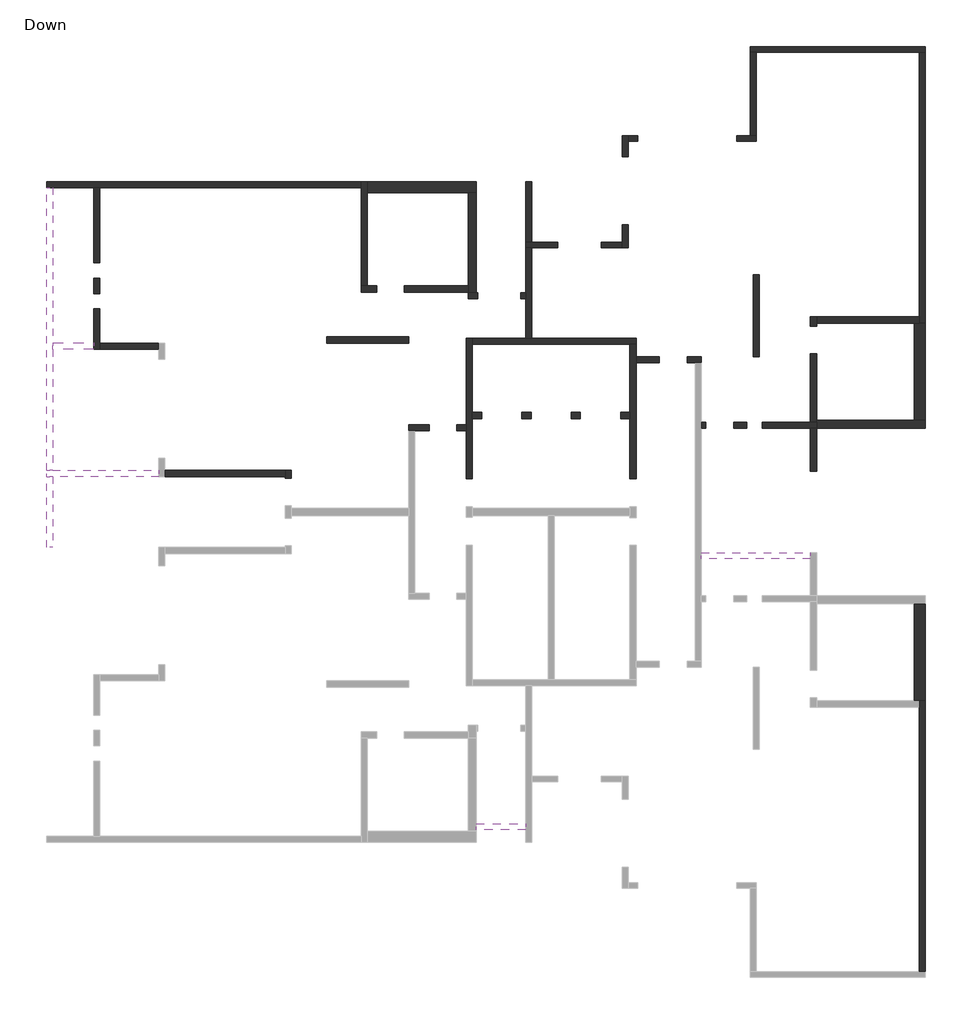
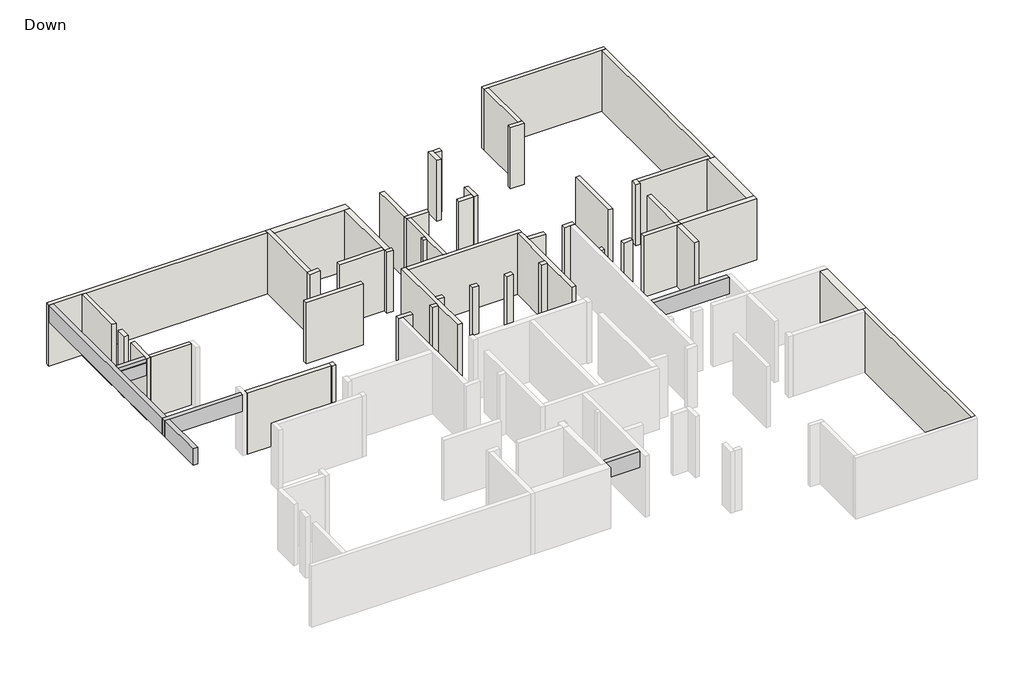
# One storey, part 2 of 2: 49 walls, 6 beams.
"""IFC4 building model written with IfcOpenShell, lengths in millimetres."""

import ifcopenshell
import ifcopenshell.guid

model = None  # the IFC model being written
_history = None  # IfcOwnerHistory: only IFC2X3 demands one
_inside = {}  # id of a spatial element -> (the spatial element, [elements in it])
_under = {}  # id of a project, library or spatial element -> (it, [spatial elements below it])
_declared = {}  # id of a project -> (the project, [libraries it declares])
_typed = {}  # id of a type object -> (the type object, [elements of that type])
_made_of = {}  # id of a material, layer set ... -> (it, [elements and type objects made of it])


def new_model(schema):
    """Start an empty IFC model of exactly this schema.

    Asked for "IFC4X3", IfcOpenShell would pick the latest addendum, in which some entities
    have other attributes; the version numbers below select the first issue.
    IFC2X3 requires an IfcOwnerHistory on every rooted entity: one is made here for all.
    """
    global model, _history
    if schema == "IFC4X3":
        model = ifcopenshell.file(schema_version=(4, 3, 0, 0))
    else:
        model = ifcopenshell.file(schema=schema)
    _inside.clear()
    _under.clear()
    _declared.clear()
    _typed.clear()
    _made_of.clear()
    _history = None
    if model.schema == "IFC2X3":
        org = make("IfcOrganization", Name="unknown")
        user = make(
            "IfcPersonAndOrganization",
            ThePerson=make("IfcPerson", FamilyName="unknown"),
            TheOrganization=org,
        )
        app = make(
            "IfcApplication",
            ApplicationDeveloper=org,
            Version="unknown",
            ApplicationFullName="unknown",
            ApplicationIdentifier="unknown",
        )
        _history = make(
            "IfcOwnerHistory",
            OwningUser=user,
            OwningApplication=app,
            ChangeAction="ADDED",
            CreationDate=0,
        )
    return model


def make(cls, **values):
    """One entity of the class cls with the attributes given. An attribute that is None is left unset."""
    return model.create_entity(
        cls, **{name: value for name, value in values.items() if value is not None}
    )


def rooted(cls, **values):
    """An entity with a GlobalId (a new one), such as an element, a storey or a relation."""
    return make(cls, GlobalId=ifcopenshell.guid.new(), OwnerHistory=_history, **values)


def si_unit(unit_type, name, prefix=None):
    """IfcSIUnit, for example si_unit("LENGTHUNIT", "METRE", prefix="MILLI")."""
    return make("IfcSIUnit", UnitType=unit_type, Prefix=prefix, Name=name)


def assignment(units):
    """IfcUnitAssignment: the units of a project."""
    return None if units is None else make("IfcUnitAssignment", Units=units)


def point(xyz):
    """IfcCartesianPoint."""
    return None if xyz is None else make("IfcCartesianPoint", Coordinates=xyz)


def direction(xyz):
    """IfcDirection."""
    return None if xyz is None else make("IfcDirection", DirectionRatios=xyz)


def frame(location, z_axis=None, x_axis=None):
    """IfcAxis2Placement3D, a coordinate frame: its origin and axes. An axis left out is left unset."""
    return make(
        "IfcAxis2Placement3D",
        Location=point(location),
        Axis=direction(z_axis),
        RefDirection=direction(x_axis),
    )


def origin():
    """The frame at (0, 0, 0) with its axes left unset."""
    return frame((0.0, 0.0, 0.0))


def place(relative_to, where):
    """IfcLocalPlacement: puts the frame where relative to a parent placement (None: the world)."""
    return make(
        "IfcLocalPlacement", PlacementRelTo=relative_to, RelativePlacement=where
    )


def context(
    kind, dimensions, precision=None, world=None, true_north=None, identifier=None
):
    """IfcGeometricRepresentationContext, for example the 3D "Model" context."""
    return make(
        "IfcGeometricRepresentationContext",
        ContextIdentifier=identifier,
        ContextType=kind,
        CoordinateSpaceDimension=dimensions,
        Precision=precision,
        WorldCoordinateSystem=world,
        TrueNorth=true_north,
    )


def project(units=None, contexts=None):
    """IfcProject with its units and contexts."""
    return rooted(
        "IfcProject",
        Name="project",
        RepresentationContexts=contexts,
        UnitsInContext=assignment(units),
    )


def spatial(cls, under=None, at=None, **own):
    """A site, building, storey or space (cls), placed at a placement, below another one or the project."""
    s = rooted(cls, ObjectPlacement=at, **own)
    if under is not None:
        _under.setdefault(under.id(), (under, []))[1].append(s)
    return s


def polyline(points):
    """IfcPolyline through the points."""
    return make("IfcPolyline", Points=[point(p) for p in points])


def outline(outer, holes=None, kind="AREA"):
    """IfcArbitraryClosedProfileDef: a profile drawn as a closed curve; with holes, ...WithVoids."""
    if holes is None:
        return make("IfcArbitraryClosedProfileDef", ProfileType=kind, OuterCurve=outer)
    return make(
        "IfcArbitraryProfileDefWithVoids",
        ProfileType=kind,
        OuterCurve=outer,
        InnerCurves=holes,
    )


def extrude(swept, where, along, depth):
    """IfcExtrudedAreaSolid: the profile swept, set in the frame where, extruded along a direction by depth."""
    return make(
        "IfcExtrudedAreaSolid",
        SweptArea=swept,
        Position=where,
        ExtrudedDirection=direction(along),
        Depth=depth,
    )


def faces_of(points, faces, orient=None, outer=None):
    """IfcFace entities. A face is a list of loops; a loop is a list of indices into points, from 0.

    orient and outer hold one flag for each loop. By default every Orientation is true, the
    first loop of a face is its IfcFaceOuterBound and the others are IfcFaceBound.
    """
    made = []
    for i, loops in enumerate(faces):
        bounds = []
        for j, loop in enumerate(loops):
            is_outer = j == 0 if outer is None else outer[i][j]
            bounds.append(
                make(
                    "IfcFaceOuterBound" if is_outer else "IfcFaceBound",
                    Bound=make("IfcPolyLoop", Polygon=[points[k] for k in loop]),
                    Orientation=True if orient is None else orient[i][j],
                )
            )
        made.append(make("IfcFace", Bounds=bounds))
    return made


def faceted_brep(points, faces, orient=None, outer=None, voids=None):
    """IfcFacetedBrep: a solid bounded by flat faces; with voids (closed shells), ...WithVoids."""
    shared = [point(p) for p in points]
    hull = make("IfcClosedShell", CfsFaces=faces_of(shared, faces, orient, outer))
    if voids is None:
        return make("IfcFacetedBrep", Outer=hull)
    return make(
        "IfcFacetedBrepWithVoids",
        Outer=hull,
        Voids=[
            make(cls, CfsFaces=faces_of(shared, fs, o, b)) for cls, fs, o, b in voids
        ],
    )


def shape(context_of_items, identifier, shape_type, items):
    """IfcShapeRepresentation: the items that make up one representation, for example the "Body"."""
    return make(
        "IfcShapeRepresentation",
        ContextOfItems=context_of_items,
        RepresentationIdentifier=identifier,
        RepresentationType=shape_type,
        Items=items,
    )


def made_of(thing, what):
    """Note that an element or type object is made of a material, layer set ...; save() writes the relation."""
    if what is not None:
        _made_of.setdefault(what.id(), (what, []))[1].append(thing)
    return thing


def element(
    cls,
    number,
    at=None,
    inside=None,
    cuts=None,
    type_object=None,
    material=None,
    context=None,
    identifier="Body",
    shape_type=None,
    held_by="IfcProductDefinitionShape",
    body=None,
    shapes=None,
    **own,
):
    """One element of the class cls, such as IfcWall. Its Tag is "e" and its number.

    at: its placement. inside: the storey or other place that contains it. cuts: it is an
    opening in that element (IfcRelVoidsElement). A single representation is given by context,
    identifier, shape_type and body (its items); several are given by shapes. held_by: the class
    of the entity that holds the representations. save() writes the other relations.
    """
    e = rooted(cls, Tag="e%d" % number, ObjectPlacement=at, **own)
    if body is not None:
        shapes = [shape(context, identifier, shape_type, body)]
    if shapes is not None:
        e.Representation = make(held_by, Representations=shapes)
    if inside is not None:
        _inside.setdefault(inside.id(), (inside, []))[1].append(e)
    if cuts is not None:
        rooted(
            "IfcRelVoidsElement", RelatingBuildingElement=cuts, RelatedOpeningElement=e
        )
    if type_object is not None:
        _typed.setdefault(type_object.id(), (type_object, []))[1].append(e)
    return made_of(e, material)


def aggregate(whole, parts):
    """IfcRelAggregates: a whole, such as a stair, and the parts it consists of."""
    return rooted("IfcRelAggregates", RelatingObject=whole, RelatedObjects=parts)


def save(model, path):
    """Write the relations noted so far, then the file.

    IfcRelAggregates (storeys below a building ...), IfcRelContainedInSpatialStructure (elements
    in a storey), IfcRelDefinesByType, IfcRelAssociatesMaterial and IfcRelDeclares: one each for
    every whole, place, type object, material and project.
    """
    for whole, parts in _under.values():
        aggregate(whole, parts)
    for where, things in _inside.values():
        rooted(
            "IfcRelContainedInSpatialStructure",
            RelatedElements=things,
            RelatingStructure=where,
        )
    for kind, things in _typed.values():
        rooted("IfcRelDefinesByType", RelatedObjects=things, RelatingType=kind)
    for what, things in _made_of.values():
        rooted("IfcRelAssociatesMaterial", RelatedObjects=things, RelatingMaterial=what)
    for by, libraries in _declared.values():
        rooted("IfcRelDeclares", RelatingContext=by, RelatedDefinitions=libraries)
    model.write(path)


model = new_model("IFC4")

# Units and contexts
model_context = context("Model", 3, world=origin())
ifc_project = project(units=[si_unit("LENGTHUNIT", "METRE", prefix="MILLI")], contexts=[model_context])

# Site, building, storey
site = spatial("IfcSite", under=ifc_project)
building = spatial("IfcBuilding", under=site)
storey = spatial("IfcBuildingStorey", under=building, Name="Down", Elevation=0.0)

# Beams
placement = place(None, origin())
element("IfcBeam", 1, ObjectType="Concrete Rectengular Beam : 20/80", at=placement, inside=storey, context=model_context, shape_type="Brep", body=[
    faceted_brep([(7776.7577342, 15926.4707233, 3000.0), (7776.7577342, 16126.4707233, 3000.0), (4344.3623691, 16126.4707233, 3000.0), (4144.3623691, 16126.4707233, 3000.0), (4144.3623691, 15926.4707233, 3000.0), (4344.3623691, 15926.4707233, 3000.0), (7776.7577342, 16126.4707233, 2810.0), (7776.7577342, 16126.4707233, 2200.0), (4344.3623691, 16126.4707233, 2200.0), (4144.3623691, 16126.4707233, 2200.0), (7776.7577342, 15926.4707233, 2200.0), (4344.3623691, 15926.4707233, 2200.0), (4144.3623691, 15926.4707233, 2200.0)], [[[0, 1, 2, 3, 4, 5]], [[1, 6, 7, 8, 9, 3, 2]], [[7, 10, 11, 12, 9, 8]], [[10, 0, 5, 4, 12, 11]], [[1, 0, 10, 7, 6]], [[4, 3, 9, 12]]]),
])
element("IfcBeam", 2, ObjectType="Concrete Rectengular Beam : 20/80", at=placement, inside=storey, context=model_context, shape_type="Brep", body=[
    faceted_brep([(4344.3623691, 25280.6199284, 3000.0), (4144.3623691, 25280.6199284, 3000.0), (4144.3623691, 16126.4707233, 3000.0), (4344.3623691, 16126.4707233, 3000.0), (4344.3623691, 20073.0459905, 3000.0), (4344.3623691, 20253.0459905, 3000.0), (4344.3623691, 25280.6199284, 2200.0), (4344.3623691, 25280.6199284, 2810.0), (4344.3623691, 16126.4707233, 2810.0), (4344.3623691, 16126.4707233, 2200.0), (4344.3623691, 20058.0459905, 2200.0), (4344.3623691, 20258.0459905, 2200.0), (4144.3623691, 25280.6199284, 2200.0), (4144.3623691, 16126.4707233, 2200.0)], [[[0, 1, 2, 3, 4, 5]], [[6, 7, 0, 5, 4, 3, 8, 9, 10, 11]], [[12, 6, 11, 10, 9, 13]], [[1, 12, 13, 2]], [[1, 0, 7, 6, 12]], [[3, 2, 13, 9, 8]]]),
])
element("IfcBeam", 3, ObjectType="Concrete Rectengular Beam : 20/80", at=placement, inside=storey, context=model_context, shape_type="SweptSolid", body=[
    extrude(outline(polyline([(20258.0459905, 2200.0), (20058.0459905, 2200.0), (20058.0459905, 2810.0), (20073.0459905, 2810.0), (20073.0459905, 3000.0), (20253.0459905, 3000.0), (20253.0459905, 2810.0), (20258.0459905, 2810.0), (20258.0459905, 2200.0)])), frame((4344.3623691, 0.0, 0.0), z_axis=(1.0, 0.0, 0.0), x_axis=(0.0, 1.0, 0.0)), (0.0, 0.0, 1.0), 1331.6661672),
])
element("IfcBeam", 4, ObjectType="Concrete Rectengular Beam : 20/80", at=placement, inside=storey, context=model_context, shape_type="SweptSolid", body=[
    extrude(outline(polyline([(4144.3623691, 15926.4707233), (4344.3623691, 15926.4707233), (4344.3623691, 13635.0363012), (4144.3623691, 13635.0363012), (4144.3623691, 15926.4707233)])), frame((0.0, 0.0, 2200.0), z_axis=(0.0, 0.0, 1.0), x_axis=(1.0, 0.0, 0.0)), (0.0, 0.0, 1.0), 800.0),
])
element("IfcBeam", 5, ObjectType="Concrete Rectengular Beam : 20/80", at=placement, inside=storey, context=model_context, shape_type="Brep", body=[
    faceted_brep([(25344.8278571, 13464.5588264, 3000.0), (25344.8278571, 13264.5588264, 3000.0), (28875.6979001, 13264.5588264, 3000.0), (28875.6979001, 13464.5588264, 3000.0), (25344.8278571, 13464.5588264, 2200.0), (28875.6979001, 13464.5588264, 2200.0), (25344.8278571, 13264.5588264, 2200.0), (28875.6979001, 13264.5588264, 2200.0), (25344.8278571, 13264.5588264, 2810.0), (28875.6979001, 13264.5588264, 2810.0)], [[[0, 1, 2, 3]], [[4, 0, 3, 5]], [[6, 4, 5, 7]], [[1, 8, 6, 7, 9, 2]], [[1, 0, 4, 6, 8]], [[3, 2, 9, 7, 5]]]),
])
element("IfcBeam", 6, ObjectType="Concrete Rectengular Beam : 20/80", at=placement, inside=storey, context=model_context, shape_type="Brep", body=[
    faceted_brep([(19662.6522503, 4492.2283899, 3000.0), (19662.6522503, 4692.2283899, 3000.0), (18051.1049523, 4692.2283899, 3000.0), (18051.1049523, 4492.2283899, 3000.0), (19662.6522503, 4492.2283899, 2200.0), (18051.1049523, 4492.2283899, 2200.0), (19662.6522503, 4692.2283899, 2200.0), (18051.1049523, 4692.2283899, 2200.0), (19662.6522503, 4692.2283899, 2810.0), (18051.1049523, 4692.2283899, 2810.0)], [[[0, 1, 2, 3]], [[4, 0, 3, 5]], [[6, 4, 5, 7]], [[1, 8, 6, 7, 9, 2]], [[1, 0, 4, 6, 8]], [[3, 2, 9, 7, 5]]]),
])

# Walls
element("IfcWall", 7, ObjectType="19", at=placement, inside=storey, context=model_context, shape_type="Brep", body=[
    faceted_brep([(32597.3840453, 29852.2723415, 0.0), (26934.7329615, 29852.2723415, 0.0), (26934.7329615, 29852.2723415, 2810.0), (26934.7329615, 29852.2723415, 3000.0), (32597.3840453, 29852.2723415, 3000.0), (32597.3840453, 29662.2723415, 0.0), (32597.3840453, 29662.2723415, 3000.0), (32407.3840453, 29662.2723415, 3000.0), (27124.7329615, 29662.2723415, 3000.0), (26934.7329615, 29662.2723415, 3000.0), (26934.7329615, 29662.2723415, 0.0), (27124.7329615, 29662.2723415, 0.0), (32407.3840453, 29662.2723415, 0.0)], [[[0, 1, 2, 3, 4]], [[5, 6, 7, 8, 9, 10, 11, 12]], [[1, 0, 5, 12, 11, 10]], [[4, 3, 9, 8, 7, 6]], [[3, 2, 1, 10, 9]], [[0, 4, 6, 5]]]),
])
element("IfcWall", 8, ObjectType="19", at=placement, inside=storey, context=model_context, shape_type="Brep", body=[
    faceted_brep([(14329.4188071, 25470.6199284, 0.0), (4143.9417549, 25470.6199284, 0.0), (4143.9417549, 25470.6199284, 3000.0), (14329.4188071, 25470.6199284, 3000.0), (14329.4188071, 25280.6199284, 0.0), (14329.4188071, 25280.6199284, 2810.0), (14329.4188071, 25280.6199284, 3000.0), (5866.0285364, 25280.6199284, 3000.0), (5676.0285364, 25280.6199284, 3000.0), (4344.3623691, 25280.6199284, 3000.0), (4143.9417549, 25280.6199284, 3000.0), (4143.9417549, 25280.6199284, 0.0), (5676.0285364, 25280.6199284, 0.0), (5866.0285364, 25280.6199284, 0.0)], [[[0, 1, 2, 3]], [[4, 5, 6, 7, 8, 9, 10, 11, 12, 13]], [[1, 0, 4, 13, 12, 11]], [[2, 1, 11, 10]], [[3, 2, 10, 9, 8, 7, 6]], [[0, 3, 6, 5, 4]]]),
])
element("IfcWall", 9, ObjectType="19", at=placement, inside=storey, context=model_context, shape_type="Brep", body=[
    faceted_brep([(5676.0285364, 25280.6199284, 0.0), (5676.0285364, 22851.8697843, 0.0), (5676.0285364, 22851.8697843, 2810.0), (5676.0285364, 22851.8697843, 3000.0), (5676.0285364, 25280.6199284, 3000.0), (5676.0285364, 25280.6199284, 2810.0), (5866.0285364, 25280.6199284, 0.0), (5866.0285364, 25280.6199284, 2810.0), (5866.0285364, 25280.6199284, 3000.0), (5866.0285364, 22851.8697843, 3000.0), (5866.0285364, 22851.8697843, 2810.0), (5866.0285364, 22851.8697843, 0.0), (5681.0285364, 22851.8697843, 3000.0)], [[[0, 1, 2, 3, 4, 5]], [[6, 7, 8, 9, 10, 11]], [[1, 0, 6, 11]], [[3, 2, 1, 11, 10, 9, 12]], [[4, 3, 12, 9, 8]], [[0, 5, 4, 8, 7, 6]]]),
])
element("IfcWall", 10, ObjectType="19", at=placement, inside=storey, context=model_context, shape_type="Brep", body=[
    faceted_brep([(5676.0285364, 22352.6390151, 0.0), (5676.0285364, 21853.4082459, 0.0), (5676.0285364, 21853.4082459, 2810.0), (5676.0285364, 21853.4082459, 3000.0), (5676.0285364, 22352.6390151, 3000.0), (5676.0285364, 22352.6390151, 2810.0), (5866.0285364, 22352.6390151, 0.0), (5866.0285364, 22352.6390151, 2810.0), (5866.0285364, 22352.6390151, 3000.0), (5866.0285364, 21853.4082459, 3000.0), (5866.0285364, 21853.4082459, 2810.0), (5866.0285364, 21853.4082459, 0.0), (5681.0285364, 21853.4082459, 3000.0), (5681.0285364, 22352.6390151, 3000.0)], [[[0, 1, 2, 3, 4, 5]], [[6, 7, 8, 9, 10, 11]], [[1, 0, 6, 11]], [[3, 2, 1, 11, 10, 9, 12]], [[4, 3, 12, 9, 8, 13]], [[0, 5, 4, 13, 8, 7, 6]]]),
])
element("IfcWall", 11, ObjectType="19", at=placement, inside=storey, context=model_context, shape_type="Brep", body=[
    faceted_brep([(5676.0285364, 21354.1774766, 0.0), (5676.0285364, 20058.0459905, 0.0), (5676.0285364, 20058.0459905, 2810.0), (5676.0285364, 20058.0459905, 3000.0), (5676.0285364, 20073.0459905, 3000.0), (5676.0285364, 20253.0459905, 3000.0), (5676.0285364, 21354.1774766, 3000.0), (5676.0285364, 21354.1774766, 2810.0), (5866.0285364, 21354.1774766, 0.0), (5866.0285364, 21354.1774766, 2810.0), (5866.0285364, 21354.1774766, 3000.0), (5866.0285364, 20248.0459905, 3000.0), (5866.0285364, 20058.0459905, 3000.0), (5866.0285364, 20058.0459905, 0.0), (5866.0285364, 20248.0459905, 0.0), (5681.0285364, 21354.1774766, 3000.0)], [[[0, 1, 2, 3, 4, 5, 6, 7]], [[8, 9, 10, 11, 12, 13, 14]], [[1, 0, 8, 14, 13]], [[6, 5, 4, 3, 12, 11, 10, 15]], [[0, 7, 6, 15, 10, 9, 8]], [[3, 2, 1, 13, 12]]]),
])
element("IfcWall", 12, ObjectType="19", at=placement, inside=storey, context=model_context, shape_type="Brep", body=[
    faceted_brep([(26934.7329615, 29662.2723415, 0.0), (26934.7329615, 26971.6500261, 0.0), (26934.7329615, 26971.6500261, 2810.0), (26934.7329615, 26971.6500261, 3000.0), (26934.7329615, 29662.2723415, 3000.0), (27124.7329615, 29662.2723415, 0.0), (27124.7329615, 29662.2723415, 2810.0), (27124.7329615, 29662.2723415, 3000.0), (27124.7329615, 26971.6500261, 3000.0), (27124.7329615, 26971.6500261, 0.0)], [[[0, 1, 2, 3, 4]], [[5, 6, 7, 8, 9]], [[1, 0, 5, 9]], [[4, 3, 8, 7]], [[0, 4, 7, 6, 5]], [[3, 2, 1, 9, 8]]]),
])
element("IfcWall", 13, ObjectType="19", at=placement, inside=storey, context=model_context, shape_type="Brep", body=[
    faceted_brep([(27124.7329615, 26971.6500261, 0.0), (26934.7329615, 26971.6500261, 0.0), (26490.0221434, 26971.6500261, 0.0), (26490.0221434, 26971.6500261, 2810.0), (26490.0221434, 26971.6500261, 3000.0), (26934.7329615, 26971.6500261, 3000.0), (27124.7329615, 26971.6500261, 3000.0), (27124.7329615, 26781.6500261, 0.0), (27124.7329615, 26781.6500261, 2810.0), (27124.7329615, 26781.6500261, 3000.0), (26490.0221434, 26781.6500261, 3000.0), (26490.0221434, 26781.6500261, 2810.0), (26490.0221434, 26781.6500261, 0.0)], [[[0, 1, 2, 3, 4, 5, 6]], [[7, 8, 9, 10, 11, 12]], [[2, 1, 0, 7, 12]], [[4, 3, 2, 12, 11, 10]], [[6, 5, 4, 10, 9]], [[0, 6, 9, 8, 7]]]),
])
element("IfcWall", 14, ObjectType="19", at=placement, inside=storey, context=model_context, shape_type="Brep", body=[
    faceted_brep([(23288.1042531, 26971.6500261, 0.0), (22974.0986592, 26971.6500261, 0.0), (22974.0986592, 26971.6500261, 3000.0), (23288.1042531, 26971.6500261, 3000.0), (23288.1042531, 26971.6500261, 2810.0), (23288.1042531, 26781.6500261, 0.0), (23288.1042531, 26781.6500261, 2810.0), (23288.1042531, 26781.6500261, 3000.0), (22974.0986592, 26781.6500261, 3000.0), (22974.0986592, 26781.6500261, 2810.0), (22974.0986592, 26781.6500261, 0.0)], [[[0, 1, 2, 3, 4]], [[5, 6, 7, 8, 9, 10]], [[1, 0, 5, 10]], [[3, 2, 8, 7]], [[0, 4, 3, 7, 6, 5]], [[2, 1, 10, 9, 8]]]),
])
element("IfcWall", 15, ObjectType="19", at=placement, inside=storey, context=model_context, shape_type="Brep", body=[
    faceted_brep([(22784.0986592, 26971.6500261, 0.0), (22784.0986592, 26281.8797734, 0.0), (22784.0986592, 26281.8797734, 2810.0), (22784.0986592, 26281.8797734, 3000.0), (22784.0986592, 26971.6500261, 3000.0), (22784.0986592, 26971.6500261, 2810.0), (22974.0986592, 26971.6500261, 0.0), (22974.0986592, 26971.6500261, 3000.0), (22974.0986592, 26781.6500261, 3000.0), (22974.0986592, 26281.8797734, 3000.0), (22974.0986592, 26281.8797734, 2810.0), (22974.0986592, 26281.8797734, 0.0), (22974.0986592, 26781.6500261, 0.0)], [[[0, 1, 2, 3, 4, 5]], [[6, 7, 8, 9, 10, 11, 12]], [[1, 0, 6, 12, 11]], [[3, 2, 1, 11, 10, 9]], [[4, 3, 9, 8, 7]], [[0, 5, 4, 7, 6]]]),
])
element("IfcWall", 16, ObjectType="19", at=placement, inside=storey, context=model_context, shape_type="Brep", body=[
    faceted_brep([(22784.6890098, 24081.620059, 0.0), (22784.6890098, 23519.8470094, 0.0), (22784.6890098, 23329.8470094, 0.0), (22784.6890098, 23329.8470094, 3000.0), (22784.6890098, 23519.8470094, 3000.0), (22784.6890098, 24081.620059, 3000.0), (22784.6890098, 24081.620059, 2810.0), (22974.6890098, 24081.620059, 0.0), (22974.6890098, 24081.620059, 2810.0), (22974.6890098, 24081.620059, 3000.0), (22974.6890098, 23329.8470094, 3000.0), (22974.6890098, 23329.8470094, 2810.0), (22974.6890098, 23329.8470094, 0.0)], [[[0, 1, 2, 3, 4, 5, 6]], [[7, 8, 9, 10, 11, 12]], [[2, 1, 0, 7, 12]], [[5, 4, 3, 10, 9]], [[0, 6, 5, 9, 8, 7]], [[3, 2, 12, 11, 10]]]),
])
element("IfcWall", 17, ObjectType="19", at=placement, inside=storey, context=model_context, shape_type="Brep", body=[
    faceted_brep([(22784.6890098, 23519.8470094, 0.0), (22104.3264087, 23519.8470094, 0.0), (22104.3264087, 23519.8470094, 2810.0), (22104.3264087, 23519.8470094, 3000.0), (22784.6890098, 23519.8470094, 3000.0), (22784.6890098, 23519.8470094, 2810.0), (22784.6890098, 23329.8470094, 0.0), (22784.6890098, 23329.8470094, 3000.0), (22104.3264087, 23329.8470094, 3000.0), (22104.3264087, 23329.8470094, 2810.0), (22104.3264087, 23329.8470094, 0.0)], [[[0, 1, 2, 3, 4, 5]], [[6, 7, 8, 9, 10]], [[1, 0, 6, 10]], [[3, 2, 1, 10, 9, 8]], [[4, 3, 8, 7]], [[0, 5, 4, 7, 6]]]),
])
element("IfcWall", 18, ObjectType="19", at=placement, inside=storey, context=model_context, shape_type="Brep", body=[
    faceted_brep([(20702.4284964, 23519.8470094, 0.0), (19852.6522503, 23519.8470094, 0.0), (19662.6522503, 23519.8470094, 0.0), (19662.6522503, 23519.8470094, 3000.0), (19852.6522503, 23519.8470094, 3000.0), (20702.4284964, 23519.8470094, 3000.0), (20702.4284964, 23519.8470094, 2810.0), (20702.4284964, 23329.8470094, 0.0), (20702.4284964, 23329.8470094, 2810.0), (20702.4284964, 23329.8470094, 3000.0), (19852.6522503, 23329.8470094, 3000.0), (19662.6522503, 23329.8470094, 3000.0), (19662.6522503, 23329.8470094, 0.0), (19852.6522503, 23329.8470094, 0.0)], [[[0, 1, 2, 3, 4, 5, 6]], [[7, 8, 9, 10, 11, 12, 13]], [[2, 1, 0, 7, 13, 12]], [[5, 4, 3, 11, 10, 9]], [[0, 6, 5, 9, 8, 7]], [[3, 2, 12, 11]]]),
])
element("IfcWall", 19, ObjectType="19", at=placement, inside=storey, context=model_context, shape_type="Brep", body=[
    faceted_brep([(19852.6522503, 23519.8470094, 0.0), (19852.6522503, 25470.811948, 0.0), (19852.6522503, 25470.811948, 2810.0), (19852.6522503, 25470.811948, 3000.0), (19852.6522503, 23519.8470094, 3000.0), (19852.6522503, 23519.8470094, 2810.0), (19662.6522503, 23519.8470094, 0.0), (19662.6522503, 23519.8470094, 3000.0), (19662.6522503, 24869.2786346, 3000.0), (19662.6522503, 25470.811948, 3000.0), (19662.6522503, 25470.811948, 2810.0), (19662.6522503, 25470.811948, 0.0)], [[[0, 1, 2, 3, 4, 5]], [[6, 7, 8, 9, 10, 11]], [[1, 0, 6, 11]], [[3, 2, 1, 11, 10, 9]], [[4, 3, 9, 8, 7]], [[0, 5, 4, 7, 6]]]),
])
element("IfcWall", 20, ObjectType="19", at=placement, inside=storey, context=model_context, shape_type="Brep", body=[
    faceted_brep([(32407.3840453, 29662.2723415, 0.0), (32407.3840453, 21099.9399072, 0.0), (32407.3840453, 20899.9399072, 0.0), (32407.3840453, 20899.9399072, 3000.0), (32407.3840453, 21099.9399072, 3000.0), (32407.3840453, 29662.2723415, 3000.0), (32407.3840453, 29662.2723415, 2810.0), (32597.3840453, 29662.2723415, 0.0), (32597.3840453, 29662.2723415, 3000.0), (32597.3840453, 20899.9399072, 3000.0), (32597.3840453, 20899.9399072, 0.0)], [[[0, 1, 2, 3, 4, 5, 6]], [[7, 8, 9, 10]], [[2, 1, 0, 7, 10]], [[5, 4, 3, 9, 8]], [[0, 6, 5, 8, 7]], [[3, 2, 10, 9]]]),
])
element("IfcWall", 21, ObjectType="19", at=placement, inside=storey, context=model_context, shape_type="Brep", body=[
    faceted_brep([(5866.0285364, 20058.0459905, 0.0), (7776.7577342, 20058.0459905, 0.0), (7776.7577342, 20058.0459905, 2810.0), (7776.7577342, 20058.0459905, 3000.0), (5866.0285364, 20058.0459905, 3000.0), (5866.0285364, 20248.0459905, 0.0), (5866.0285364, 20248.0459905, 2810.0), (5866.0285364, 20248.0459905, 3000.0), (7776.7577342, 20248.0459905, 3000.0), (7776.7577342, 20248.0459905, 0.0)], [[[0, 1, 2, 3, 4]], [[5, 6, 7, 8, 9]], [[1, 0, 5, 9]], [[4, 3, 8, 7]], [[0, 4, 7, 6, 5]], [[3, 2, 1, 9, 8]]]),
])
element("IfcWall", 22, ObjectType="19", at=placement, inside=storey, context=model_context, shape_type="Brep", body=[
    faceted_brep([(11878.6856136, 16126.4707233, 0.0), (11878.6856136, 15926.4707233, 0.0), (11878.6856136, 15877.7643004, 0.0), (11878.6856136, 15877.7643004, 2810.0), (11878.6856136, 15877.7643004, 3000.0), (11878.6856136, 15926.4707233, 3000.0), (11878.6856136, 16126.4707233, 3000.0), (12068.6856136, 16126.4707233, 0.0), (12068.6856136, 16126.4707233, 2810.0), (12068.6856136, 16126.4707233, 3000.0), (12068.6856136, 15877.7643004, 3000.0), (12068.6856136, 15877.7643004, 2810.0), (12068.6856136, 15877.7643004, 0.0)], [[[0, 1, 2, 3, 4, 5, 6]], [[7, 8, 9, 10, 11, 12]], [[2, 1, 0, 7, 12]], [[4, 3, 2, 12, 11, 10]], [[6, 5, 4, 10, 9]], [[0, 6, 9, 8, 7]]]),
])
element("IfcWall", 23, ObjectType="19", at=placement, inside=storey, context=model_context, shape_type="Brep", body=[
    faceted_brep([(17801.1049523, 21688.6523235, 0.0), (18101.9290458, 21688.6523235, 0.0), (18101.9290458, 21688.6523235, 2810.0), (18101.9290458, 21688.6523235, 3000.0), (17801.1049523, 21688.6523235, 3000.0), (17801.1049523, 21688.6523235, 2810.0), (17801.1049523, 21878.6523235, 0.0), (17801.1049523, 21878.6523235, 3000.0), (18051.1049523, 21878.6523235, 3000.0), (18101.9290458, 21878.6523235, 3000.0), (18101.9290458, 21878.6523235, 2810.0), (18101.9290458, 21878.6523235, 0.0), (18051.1049523, 21878.6523235, 0.0)], [[[0, 1, 2, 3, 4, 5]], [[6, 7, 8, 9, 10, 11, 12]], [[1, 0, 6, 12, 11]], [[3, 2, 1, 11, 10, 9]], [[4, 3, 9, 8, 7]], [[0, 5, 4, 7, 6]]]),
])
element("IfcWall", 24, ObjectType="19", at=placement, inside=storey, context=model_context, shape_type="Brep", body=[
    faceted_brep([(19501.7092875, 21688.6523235, 0.0), (19662.6522503, 21688.6523235, 0.0), (19662.6522503, 21688.6523235, 2810.0), (19662.6522503, 21688.6523235, 3000.0), (19501.7092875, 21688.6523235, 3000.0), (19501.7092875, 21688.6523235, 2810.0), (19501.7092875, 21878.6523235, 0.0), (19501.7092875, 21878.6523235, 2810.0), (19501.7092875, 21878.6523235, 3000.0), (19662.6522503, 21878.6523235, 3000.0), (19662.6522503, 21878.6523235, 2810.0), (19662.6522503, 21878.6523235, 0.0)], [[[0, 1, 2, 3, 4, 5]], [[6, 7, 8, 9, 10, 11]], [[1, 0, 6, 11]], [[4, 3, 9, 8]], [[0, 5, 4, 8, 7, 6]], [[3, 2, 1, 11, 10, 9]]]),
])
element("IfcWall", 25, ObjectType="19", at=placement, inside=storey, context=model_context, shape_type="Brep", body=[
    faceted_brep([(19662.6522503, 23329.8470094, 0.0), (19662.6522503, 21878.6523235, 0.0), (19662.6522503, 21688.6523235, 0.0), (19662.6522503, 20409.5793039, 0.0), (19662.6522503, 20409.5793039, 2810.0), (19662.6522503, 20409.5793039, 3000.0), (19662.6522503, 21688.6523235, 3000.0), (19662.6522503, 21878.6523235, 3000.0), (19662.6522503, 23329.8470094, 3000.0), (19852.6522503, 23329.8470094, 0.0), (19852.6522503, 23329.8470094, 2810.0), (19852.6522503, 23329.8470094, 3000.0), (19852.6522503, 20409.5793039, 3000.0), (19852.6522503, 20409.5793039, 2810.0), (19852.6522503, 20409.5793039, 0.0)], [[[0, 1, 2, 3, 4, 5, 6, 7, 8]], [[9, 10, 11, 12, 13, 14]], [[3, 2, 1, 0, 9, 14]], [[8, 7, 6, 5, 12, 11]], [[0, 8, 11, 10, 9]], [[5, 4, 3, 14, 13, 12]]]),
])
element("IfcWall", 26, ObjectType="19", at=placement, inside=storey, context=model_context, shape_type="Brep", body=[
    faceted_brep([(32597.3840453, -100.765317, 0.0), (32597.3840453, 8661.5671173, 0.0), (32597.3840453, 8661.5671173, 3000.0), (32597.3840453, -100.765317, 3000.0), (32407.3840453, -100.765317, 0.0), (32407.3840453, -100.765317, 2810.0), (32407.3840453, -100.765317, 3000.0), (32407.3840453, 8461.5671173, 3000.0), (32407.3840453, 8661.5671173, 3000.0), (32407.3840453, 8661.5671173, 0.0), (32407.3840453, 8461.5671173, 0.0)], [[[0, 1, 2, 3]], [[4, 5, 6, 7, 8, 9, 10]], [[1, 0, 4, 10, 9]], [[3, 2, 8, 7, 6]], [[0, 3, 6, 5, 4]], [[2, 1, 9, 8]]]),
])
element("IfcWall", 27, ObjectType="20", at=placement, inside=storey, context=model_context, shape_type="Brep", body=[
    faceted_brep([(14529.4188071, 22100.4193798, 0.0), (14529.4188071, 25120.7159382, 0.0), (14529.4188071, 25470.6199284, 0.0), (14529.4188071, 25470.6199284, 3000.0), (14529.4188071, 25120.7159382, 3000.0), (14529.4188071, 22100.4193798, 3000.0), (14529.4188071, 22100.4193798, 2810.0), (14329.4188071, 22100.4193798, 0.0), (14329.4188071, 22100.4193798, 3000.0), (14329.4188071, 25280.6199284, 3000.0), (14329.4188071, 25470.6199284, 3000.0), (14329.4188071, 25470.6199284, 0.0), (14329.4188071, 25280.6199284, 0.0)], [[[0, 1, 2, 3, 4, 5, 6]], [[7, 8, 9, 10, 11, 12]], [[2, 1, 0, 7, 12, 11]], [[5, 4, 3, 10, 9, 8]], [[3, 2, 11, 10]], [[0, 6, 5, 8, 7]]]),
])
element("IfcWall", 28, ObjectType="20", at=placement, inside=storey, context=model_context, shape_type="Brep", body=[
    faceted_brep([(29076.6368672, 20899.9399072, 0.0), (32247.3840453, 20899.9399072, 0.0), (32407.3840453, 20899.9399072, 0.0), (32407.3840453, 20899.9399072, 3000.0), (32247.3840453, 20899.9399072, 3000.0), (29076.6368672, 20899.9399072, 3000.0), (29076.6368672, 20899.9399072, 2810.0), (29076.6368672, 21099.9399072, 0.0), (29076.6368672, 21099.9399072, 3000.0), (32407.3840453, 21099.9399072, 3000.0), (32407.3840453, 21099.9399072, 2810.0), (32407.3840453, 21099.9399072, 0.0)], [[[0, 1, 2, 3, 4, 5, 6]], [[7, 8, 9, 10, 11]], [[2, 1, 0, 7, 11]], [[5, 4, 3, 9, 8]], [[3, 2, 11, 10, 9]], [[0, 6, 5, 8, 7]]]),
])
element("IfcWall", 29, ObjectType="20", at=placement, inside=storey, context=model_context, shape_type="Brep", body=[
    faceted_brep([(7966.7577342, 15926.4707233, 0.0), (11878.6856136, 15926.4707233, 0.0), (11878.6856136, 15926.4707233, 3000.0), (7966.7577342, 15926.4707233, 3000.0), (7966.7577342, 16126.4707233, 0.0), (7966.7577342, 16126.4707233, 2810.0), (7966.7577342, 16126.4707233, 3000.0), (11878.6856136, 16126.4707233, 3000.0), (11878.6856136, 16126.4707233, 0.0)], [[[0, 1, 2, 3]], [[4, 5, 6, 7, 8]], [[1, 0, 4, 8]], [[3, 2, 7, 6]], [[0, 3, 6, 5, 4]], [[2, 1, 8, 7]]]),
])
element("IfcWall", 30, ObjectType="20", at=placement, inside=storey, context=model_context, shape_type="Brep", body=[
    faceted_brep([(14329.4188071, 21900.4193798, 0.0), (14830.1280269, 21900.4193798, 0.0), (14830.1280269, 21900.4193798, 2810.0), (14830.1280269, 21900.4193798, 3000.0), (14329.4188071, 21900.4193798, 3000.0), (14329.4188071, 21900.4193798, 2810.0), (14329.4188071, 22100.4193798, 0.0), (14329.4188071, 22100.4193798, 3000.0), (14529.4188071, 22100.4193798, 3000.0), (14830.1280269, 22100.4193798, 3000.0), (14830.1280269, 22100.4193798, 2810.0), (14830.1280269, 22100.4193798, 0.0), (14529.4188071, 22100.4193798, 0.0)], [[[0, 1, 2, 3, 4, 5]], [[6, 7, 8, 9, 10, 11, 12]], [[1, 0, 6, 12, 11]], [[3, 2, 1, 11, 10, 9]], [[4, 3, 9, 8, 7]], [[0, 5, 4, 7, 6]]]),
])
element("IfcWall", 31, ObjectType="20", at=placement, inside=storey, context=model_context, shape_type="Brep", body=[
    faceted_brep([(15730.1380159, 21900.4193798, 0.0), (17801.1049523, 21900.4193798, 0.0), (17801.1049523, 21900.4193798, 2810.0), (17801.1049523, 21900.4193798, 3000.0), (15730.1380159, 21900.4193798, 3000.0), (15730.1380159, 21900.4193798, 2810.0), (15730.1380159, 22100.4193798, 0.0), (15730.1380159, 22100.4193798, 2810.0), (15730.1380159, 22100.4193798, 3000.0), (17801.1049523, 22100.4193798, 3000.0), (17801.1049523, 22100.4193798, 2810.0), (17801.1049523, 22100.4193798, 0.0)], [[[0, 1, 2, 3, 4, 5]], [[6, 7, 8, 9, 10, 11]], [[1, 0, 6, 11]], [[4, 3, 9, 8]], [[0, 5, 4, 8, 7, 6]], [[3, 2, 1, 11, 10, 9]]]),
])
element("IfcWall", 32, ObjectType="20", at=placement, inside=storey, context=model_context, shape_type="Brep", body=[
    faceted_brep([(13218.5807289, 20248.6363411, 0.0), (15869.904273, 20248.6363411, 0.0), (15869.904273, 20248.6363411, 2810.0), (15869.904273, 20248.6363411, 3000.0), (13218.5807289, 20248.6363411, 3000.0), (13218.5807289, 20248.6363411, 2810.0), (13218.5807289, 20448.6363411, 0.0), (13218.5807289, 20448.6363411, 2810.0), (13218.5807289, 20448.6363411, 3000.0), (15869.904273, 20448.6363411, 3000.0), (15869.904273, 20448.6363411, 2810.0), (15869.904273, 20448.6363411, 0.0)], [[[0, 1, 2, 3, 4, 5]], [[6, 7, 8, 9, 10, 11]], [[1, 0, 6, 11]], [[3, 2, 1, 11, 10, 9]], [[4, 3, 9, 8]], [[0, 5, 4, 8, 7, 6]]]),
])
element("IfcWall", 33, ObjectType="20", at=placement, inside=storey, context=model_context, shape_type="Brep", body=[
    faceted_brep([(15871.0829765, 17407.9011498, 0.0), (16071.0829765, 17407.9011498, 0.0), (16530.6174885, 17407.9011498, 0.0), (16530.6174885, 17407.9011498, 2810.0), (16530.6174885, 17407.9011498, 3000.0), (16071.0829765, 17407.9011498, 3000.0), (15871.0829765, 17407.9011498, 3000.0), (15871.0829765, 17607.9011498, 0.0), (15871.0829765, 17607.9011498, 2810.0), (15871.0829765, 17607.9011498, 3000.0), (16530.6174885, 17607.9011498, 3000.0), (16530.6174885, 17607.9011498, 2810.0), (16530.6174885, 17607.9011498, 0.0)], [[[0, 1, 2, 3, 4, 5, 6]], [[7, 8, 9, 10, 11, 12]], [[2, 1, 0, 7, 12]], [[4, 3, 2, 12, 11, 10]], [[6, 5, 4, 10, 9]], [[0, 6, 9, 8, 7]]]),
])
element("IfcWall", 34, ObjectType="20", at=placement, inside=storey, context=model_context, shape_type="Brep", body=[
    faceted_brep([(17430.6274775, 17407.9011498, 0.0), (17731.3366974, 17407.9011498, 0.0), (17731.3366974, 17407.9011498, 2810.0), (17731.3366974, 17407.9011498, 3000.0), (17430.6274775, 17407.9011498, 3000.0), (17430.6274775, 17407.9011498, 2810.0), (17430.6274775, 17607.9011498, 0.0), (17430.6274775, 17607.9011498, 2810.0), (17430.6274775, 17607.9011498, 3000.0), (17731.3366974, 17607.9011498, 3000.0), (17731.3366974, 17607.9011498, 2810.0), (17731.3366974, 17607.9011498, 0.0)], [[[0, 1, 2, 3, 4, 5]], [[6, 7, 8, 9, 10, 11]], [[1, 0, 6, 11]], [[4, 3, 9, 8]], [[0, 5, 4, 8, 7, 6]], [[3, 2, 1, 11, 10, 9]]]),
])
element("IfcWall", 35, ObjectType="20", at=placement, inside=storey, context=model_context, shape_type="Brep", body=[
    faceted_brep([(17931.3366974, 15852.9011498, 0.0), (17931.3366974, 17808.1408861, 0.0), (17931.3366974, 18008.1408861, 0.0), (17931.3366974, 20209.5793039, 0.0), (17931.3366974, 20409.5793039, 0.0), (17931.3366974, 20409.5793039, 3000.0), (17931.3366974, 20209.5793039, 3000.0), (17931.3366974, 18008.1408861, 3000.0), (17931.3366974, 17808.1408861, 3000.0), (17931.3366974, 15852.9011498, 3000.0), (17931.3366974, 15852.9011498, 2810.0), (17731.3366974, 15852.9011498, 0.0), (17731.3366974, 15852.9011498, 2810.0), (17731.3366974, 15852.9011498, 3000.0), (17731.3366974, 17407.9011498, 3000.0), (17731.3366974, 17607.9011498, 3000.0), (17731.3366974, 20409.5793039, 3000.0), (17731.3366974, 20409.5793039, 2810.0), (17731.3366974, 20409.5793039, 0.0), (17731.3366974, 17607.9011498, 0.0), (17731.3366974, 17407.9011498, 0.0)], [[[0, 1, 2, 3, 4, 5, 6, 7, 8, 9, 10]], [[11, 12, 13, 14, 15, 16, 17, 18, 19, 20]], [[4, 3, 2, 1, 0, 11, 20, 19, 18]], [[9, 8, 7, 6, 5, 16, 15, 14, 13]], [[0, 10, 9, 13, 12, 11]], [[5, 4, 18, 17, 16]]]),
])
element("IfcWall", 36, ObjectType="20", at=placement, inside=storey, context=model_context, shape_type="Brep", body=[
    faceted_brep([(17931.3366974, 20209.5793039, 0.0), (23033.0448184, 20209.5793039, 0.0), (23233.0448184, 20209.5793039, 0.0), (23233.0448184, 20209.5793039, 3000.0), (23033.0448184, 20209.5793039, 3000.0), (17931.3366974, 20209.5793039, 3000.0), (17931.3366974, 20409.5793039, 0.0), (17931.3366974, 20409.5793039, 3000.0), (19662.6522503, 20409.5793039, 3000.0), (19852.6522503, 20409.5793039, 3000.0), (23233.0448184, 20409.5793039, 3000.0), (23233.0448184, 20409.5793039, 2810.0), (23233.0448184, 20409.5793039, 0.0), (19852.6522503, 20409.5793039, 0.0), (19662.6522503, 20409.5793039, 0.0)], [[[0, 1, 2, 3, 4, 5]], [[6, 7, 8, 9, 10, 11, 12, 13, 14]], [[2, 1, 0, 6, 14, 13, 12]], [[5, 4, 3, 10, 9, 8, 7]], [[0, 5, 7, 6]], [[3, 2, 12, 11, 10]]]),
])
element("IfcWall", 37, ObjectType="20", at=placement, inside=storey, context=model_context, shape_type="Brep", body=[
    faceted_brep([(23233.0448184, 19609.0998313, 0.0), (23984.8178681, 19609.0998313, 0.0), (23984.8178681, 19609.0998313, 2810.0), (23984.8178681, 19609.0998313, 3000.0), (23233.0448184, 19609.0998313, 3000.0), (23233.0448184, 19609.0998313, 2810.0), (23233.0448184, 19809.0998313, 0.0), (23233.0448184, 19809.0998313, 2810.0), (23233.0448184, 19809.0998313, 3000.0), (23984.8178681, 19809.0998313, 3000.0), (23984.8178681, 19809.0998313, 2810.0), (23984.8178681, 19809.0998313, 0.0)], [[[0, 1, 2, 3, 4, 5]], [[6, 7, 8, 9, 10, 11]], [[1, 0, 6, 11]], [[3, 2, 1, 11, 10, 9]], [[4, 3, 9, 8]], [[0, 5, 4, 8, 7, 6]]]),
])
element("IfcWall", 38, ObjectType="20", at=placement, inside=storey, context=model_context, shape_type="Brep", body=[
    faceted_brep([(24884.8278571, 19609.0998313, 0.0), (25144.8278571, 19609.0998313, 0.0), (25344.8278571, 19609.0998313, 0.0), (25344.8278571, 19609.0998313, 3000.0), (25144.8278571, 19609.0998313, 3000.0), (24884.8278571, 19609.0998313, 3000.0), (24884.8278571, 19609.0998313, 2810.0), (24884.8278571, 19809.0998313, 0.0), (24884.8278571, 19809.0998313, 2810.0), (24884.8278571, 19809.0998313, 3000.0), (25344.8278571, 19809.0998313, 3000.0), (25344.8278571, 19809.0998313, 2810.0), (25344.8278571, 19809.0998313, 0.0)], [[[0, 1, 2, 3, 4, 5, 6]], [[7, 8, 9, 10, 11, 12]], [[2, 1, 0, 7, 12]], [[5, 4, 3, 10, 9]], [[0, 6, 5, 9, 8, 7]], [[3, 2, 12, 11, 10]]]),
])
element("IfcWall", 39, ObjectType="20", at=placement, inside=storey, context=model_context, shape_type="Brep", body=[
    faceted_brep([(23233.0448184, 15856.5875947, 0.0), (23233.0448184, 19609.0998313, 0.0), (23233.0448184, 19809.0998313, 0.0), (23233.0448184, 20209.5793039, 0.0), (23233.0448184, 20209.5793039, 3000.0), (23233.0448184, 19809.0998313, 3000.0), (23233.0448184, 19609.0998313, 3000.0), (23233.0448184, 15856.5875947, 3000.0), (23233.0448184, 15856.5875947, 2810.0), (23033.0448184, 15856.5875947, 0.0), (23033.0448184, 15856.5875947, 2810.0), (23033.0448184, 15856.5875947, 3000.0), (23033.0448184, 17808.1408861, 3000.0), (23033.0448184, 18008.1408861, 3000.0), (23033.0448184, 20209.5793039, 3000.0), (23033.0448184, 20209.5793039, 0.0), (23033.0448184, 18008.1408861, 0.0), (23033.0448184, 17808.1408861, 0.0)], [[[0, 1, 2, 3, 4, 5, 6, 7, 8]], [[9, 10, 11, 12, 13, 14, 15, 16, 17]], [[3, 2, 1, 0, 9, 17, 16, 15]], [[7, 6, 5, 4, 14, 13, 12, 11]], [[0, 8, 7, 11, 10, 9]], [[4, 3, 15, 14]]]),
])
element("IfcWall", 40, ObjectType="20", at=placement, inside=storey, context=model_context, shape_type="Brep", body=[
    faceted_brep([(23033.0448184, 18008.1408861, 0.0), (22733.2745657, 18008.1408861, 0.0), (22733.2745657, 18008.1408861, 2810.0), (22733.2745657, 18008.1408861, 3000.0), (23033.0448184, 18008.1408861, 3000.0), (23033.0448184, 17808.1408861, 0.0), (23033.0448184, 17808.1408861, 2810.0), (23033.0448184, 17808.1408861, 3000.0), (22733.2745657, 17808.1408861, 3000.0), (22733.2745657, 17808.1408861, 2810.0), (22733.2745657, 17808.1408861, 0.0)], [[[0, 1, 2, 3, 4]], [[5, 6, 7, 8, 9, 10]], [[1, 0, 5, 10]], [[3, 2, 1, 10, 9, 8]], [[4, 3, 8, 7]], [[0, 4, 7, 6, 5]]]),
])
element("IfcWall", 41, ObjectType="20", at=placement, inside=storey, context=model_context, shape_type="Brep", body=[
    faceted_brep([(21433.0248404, 18008.1408861, 0.0), (21132.3156206, 18008.1408861, 0.0), (21132.3156206, 18008.1408861, 2810.0), (21132.3156206, 18008.1408861, 3000.0), (21433.0248404, 18008.1408861, 3000.0), (21433.0248404, 18008.1408861, 2810.0), (21433.0248404, 17808.1408861, 0.0), (21433.0248404, 17808.1408861, 2810.0), (21433.0248404, 17808.1408861, 3000.0), (21132.3156206, 17808.1408861, 3000.0), (21132.3156206, 17808.1408861, 2810.0), (21132.3156206, 17808.1408861, 0.0)], [[[0, 1, 2, 3, 4, 5]], [[6, 7, 8, 9, 10, 11]], [[1, 0, 6, 11]], [[3, 2, 1, 11, 10, 9]], [[4, 3, 9, 8]], [[0, 5, 4, 8, 7, 6]]]),
])
element("IfcWall", 42, ObjectType="20", at=placement, inside=storey, context=model_context, shape_type="Brep", body=[
    faceted_brep([(19832.0658953, 18008.1408861, 0.0), (19531.3566754, 18008.1408861, 0.0), (19531.3566754, 18008.1408861, 2810.0), (19531.3566754, 18008.1408861, 3000.0), (19832.0658953, 18008.1408861, 3000.0), (19832.0658953, 18008.1408861, 2810.0), (19832.0658953, 17808.1408861, 0.0), (19832.0658953, 17808.1408861, 2810.0), (19832.0658953, 17808.1408861, 3000.0), (19531.3566754, 17808.1408861, 3000.0), (19531.3566754, 17808.1408861, 2810.0), (19531.3566754, 17808.1408861, 0.0)], [[[0, 1, 2, 3, 4, 5]], [[6, 7, 8, 9, 10, 11]], [[1, 0, 6, 11]], [[3, 2, 1, 11, 10, 9]], [[4, 3, 9, 8]], [[0, 5, 4, 8, 7, 6]]]),
])
element("IfcWall", 43, ObjectType="20", at=placement, inside=storey, context=model_context, shape_type="Brep", body=[
    faceted_brep([(18231.1069501, 18008.1408861, 0.0), (17931.3366974, 18008.1408861, 0.0), (17931.3366974, 18008.1408861, 3000.0), (18231.1069501, 18008.1408861, 3000.0), (18231.1069501, 18008.1408861, 2810.0), (18231.1069501, 17808.1408861, 0.0), (18231.1069501, 17808.1408861, 2810.0), (18231.1069501, 17808.1408861, 3000.0), (17931.3366974, 17808.1408861, 3000.0), (17931.3366974, 17808.1408861, 2810.0), (17931.3366974, 17808.1408861, 0.0)], [[[0, 1, 2, 3, 4]], [[5, 6, 7, 8, 9, 10]], [[1, 0, 5, 10]], [[3, 2, 8, 7]], [[0, 4, 3, 7, 6, 5]], [[2, 1, 10, 9, 8]]]),
])
element("IfcWall", 44, ObjectType="20", at=placement, inside=storey, context=model_context, shape_type="Brep", body=[
    faceted_brep([(25344.8278571, 17488.3726312, 0.0), (25494.7169791, 17488.3726312, 0.0), (25494.7169791, 17488.3726312, 2810.0), (25494.7169791, 17488.3726312, 3000.0), (25344.8278571, 17488.3726312, 3000.0), (25344.8278571, 17488.3726312, 2810.0), (25344.8278571, 17688.3726312, 0.0), (25344.8278571, 17688.3726312, 2810.0), (25344.8278571, 17688.3726312, 3000.0), (25494.7169791, 17688.3726312, 3000.0), (25494.7169791, 17688.3726312, 2810.0), (25494.7169791, 17688.3726312, 0.0)], [[[0, 1, 2, 3, 4, 5]], [[6, 7, 8, 9, 10, 11]], [[1, 0, 6, 11]], [[3, 2, 1, 11, 10, 9]], [[4, 3, 9, 8]], [[0, 5, 4, 8, 7, 6]]]),
])
element("IfcWall", 45, ObjectType="20", at=placement, inside=storey, context=model_context, shape_type="Brep", body=[
    faceted_brep([(26394.7269681, 17488.3726312, 0.0), (26824.6140922, 17488.3726312, 0.0), (26824.6140922, 17488.3726312, 2810.0), (26824.6140922, 17488.3726312, 3000.0), (26394.7269681, 17488.3726312, 3000.0), (26394.7269681, 17488.3726312, 2810.0), (26394.7269681, 17688.3726312, 0.0), (26394.7269681, 17688.3726312, 2810.0), (26394.7269681, 17688.3726312, 3000.0), (26824.6140922, 17688.3726312, 3000.0), (26824.6140922, 17688.3726312, 2810.0), (26824.6140922, 17688.3726312, 0.0)], [[[0, 1, 2, 3, 4, 5]], [[6, 7, 8, 9, 10, 11]], [[1, 0, 6, 11]], [[3, 2, 1, 11, 10, 9]], [[4, 3, 9, 8]], [[0, 5, 4, 8, 7, 6]]]),
])
element("IfcWall", 46, ObjectType="20", at=placement, inside=storey, context=model_context, shape_type="Brep", body=[
    faceted_brep([(27326.5020155, 17488.3726312, 0.0), (28875.6979001, 17488.3726312, 0.0), (29075.6979001, 17488.3726312, 0.0), (29075.6979001, 17488.3726312, 3000.0), (28875.6979001, 17488.3726312, 3000.0), (27326.5020155, 17488.3726312, 3000.0), (27326.5020155, 17488.3726312, 2810.0), (27326.5020155, 17688.3726312, 0.0), (27326.5020155, 17688.3726312, 2810.0), (27326.5020155, 17688.3726312, 3000.0), (28876.6368672, 17688.3726312, 3000.0), (29075.6979001, 17688.3726312, 3000.0), (29075.6979001, 17688.3726312, 0.0), (28876.6368672, 17688.3726312, 0.0), (29075.6979001, 17497.7822806, 0.0), (29075.6979001, 17497.7822806, 3000.0)], [[[0, 1, 2, 3, 4, 5, 6]], [[7, 8, 9, 10, 11, 12, 13]], [[2, 1, 0, 7, 13, 12, 14]], [[5, 4, 3, 15, 11, 10, 9]], [[0, 6, 5, 9, 8, 7]], [[3, 2, 14, 12, 11, 15]]]),
])
element("IfcWall", 47, ObjectType="20", at=placement, inside=storey, context=model_context, shape_type="Brep", body=[
    faceted_brep([(28875.6979001, 17488.3726312, 0.0), (28875.6979001, 16095.8843683, 0.0), (28875.6979001, 16095.8843683, 3000.0), (28875.6979001, 16296.9481981, 3000.0), (28875.6979001, 17488.3726312, 3000.0), (28875.6979001, 17488.3726312, 2810.0), (29075.6979001, 17488.3726312, 0.0), (29075.6979001, 17488.3726312, 3000.0), (29075.6979001, 16095.8843683, 3000.0), (29075.6979001, 16095.8843683, 0.0)], [[[0, 1, 2, 3, 4, 5]], [[6, 7, 8, 9]], [[1, 0, 6, 9]], [[2, 1, 9, 8]], [[4, 3, 2, 8, 7]], [[0, 5, 4, 7, 6]]]),
])
element("IfcWall", 48, ObjectType="20", at=placement, inside=storey, context=model_context, shape_type="Brep", body=[
    faceted_brep([(28876.6368672, 21099.9399072, 0.0), (28876.6368672, 20799.2306873, 0.0), (28876.6368672, 20799.2306873, 2810.0), (28876.6368672, 20799.2306873, 3000.0), (28876.6368672, 21099.9399072, 3000.0), (28876.6368672, 21099.9399072, 2810.0), (29076.6368672, 21099.9399072, 0.0), (29076.6368672, 21099.9399072, 3000.0), (29076.6368672, 20899.9399072, 3000.0), (29076.6368672, 20799.2306873, 3000.0), (29076.6368672, 20799.2306873, 2810.0), (29076.6368672, 20799.2306873, 0.0), (29076.6368672, 20899.9399072, 0.0)], [[[0, 1, 2, 3, 4, 5]], [[6, 7, 8, 9, 10, 11, 12]], [[1, 0, 6, 12, 11]], [[3, 2, 1, 11, 10, 9]], [[4, 3, 9, 8, 7]], [[0, 5, 4, 7, 6]]]),
])
element("IfcWall", 49, ObjectType="20", at=placement, inside=storey, context=model_context, shape_type="Brep", body=[
    faceted_brep([(28876.6368672, 19899.2206983, 0.0), (28876.6368672, 17688.3726312, 0.0), (28876.6368672, 17688.3726312, 2810.0), (28876.6368672, 17688.3726312, 3000.0), (28876.6368672, 19899.2206983, 3000.0), (28876.6368672, 19899.2206983, 2810.0), (29076.6368672, 19899.2206983, 0.0), (29076.6368672, 19899.2206983, 2810.0), (29076.6368672, 19899.2206983, 3000.0), (29076.6368672, 17747.7822806, 3000.0), (29076.6368672, 17747.7822806, 2810.0), (29076.6368672, 17747.7822806, 0.0), (29075.6979001, 17747.7822806, 0.0), (29075.6979001, 17688.3726312, 0.0), (29075.6979001, 17688.3726312, 3000.0), (29075.6979001, 17747.7822806, 3000.0)], [[[0, 1, 2, 3, 4, 5]], [[6, 7, 8, 9, 10, 11]], [[1, 0, 6, 11, 12, 13]], [[4, 3, 14, 15, 9, 8]], [[0, 5, 4, 8, 7, 6]], [[3, 2, 1, 13, 14]], [[13, 12, 15, 14]], [[12, 11, 10, 9, 15]]]),
])
element("IfcWall", 50, ObjectType="20", at=placement, inside=storey, context=model_context, shape_type="Brep", body=[
    faceted_brep([(27225.7927957, 19808.1608642, 0.0), (27225.7927957, 22459.4844083, 0.0), (27225.7927957, 22459.4844083, 2810.0), (27225.7927957, 22459.4844083, 3000.0), (27225.7927957, 19808.1608642, 3000.0), (27225.7927957, 19808.1608642, 2810.0), (27025.7927957, 19808.1608642, 0.0), (27025.7927957, 19808.1608642, 2810.0), (27025.7927957, 19808.1608642, 3000.0), (27025.7927957, 22459.4844083, 3000.0), (27025.7927957, 22459.4844083, 2810.0), (27025.7927957, 22459.4844083, 0.0)], [[[0, 1, 2, 3, 4, 5]], [[6, 7, 8, 9, 10, 11]], [[1, 0, 6, 11]], [[3, 2, 1, 11, 10, 9]], [[4, 3, 9, 8]], [[0, 5, 4, 8, 7, 6]]]),
])
element("IfcWall", 51, ObjectType="25", at=placement, inside=storey, context=model_context, shape_type="Brep", body=[
    faceted_brep([(18051.1049523, 21878.6523235, 0.0), (18051.1049523, 25120.7159382, 0.0), (18051.1049523, 25120.7159382, 3000.0), (18051.1049523, 24869.2786346, 3000.0), (18051.1049523, 21878.6523235, 3000.0), (18051.1049523, 21878.6523235, 2810.0), (17801.1049523, 21878.6523235, 0.0), (17801.1049523, 21878.6523235, 3000.0), (17801.1049523, 21900.4193798, 3000.0), (17801.1049523, 22100.4193798, 3000.0), (17801.1049523, 25120.7159382, 3000.0), (17801.1049523, 25120.7159382, 2810.0), (17801.1049523, 25120.7159382, 0.0), (17801.1049523, 22100.4193798, 0.0), (17801.1049523, 21900.4193798, 0.0)], [[[0, 1, 2, 3, 4, 5]], [[6, 7, 8, 9, 10, 11, 12, 13, 14]], [[1, 0, 6, 14, 13, 12]], [[4, 3, 2, 10, 9, 8, 7]], [[2, 1, 12, 11, 10]], [[0, 5, 4, 7, 6]]]),
])
element("IfcWall", 52, ObjectType="25", at=placement, inside=storey, context=model_context, shape_type="Brep", body=[
    faceted_brep([(29075.6979001, 17497.7822806, 0.0), (32597.3840453, 17497.7822806, 0.0), (32597.3840453, 17497.7822806, 3000.0), (29075.6979001, 17497.7822806, 3000.0), (29075.6979001, 17747.7822806, 0.0), (29075.6979001, 17747.7822806, 3000.0), (29076.6368672, 17747.7822806, 3000.0), (32247.3840453, 17747.7822806, 3000.0), (32597.3840453, 17747.7822806, 3000.0), (32597.3840453, 17747.7822806, 0.0), (32247.3840453, 17747.7822806, 0.0), (29076.6368672, 17747.7822806, 0.0), (29075.6979001, 17688.3726312, 0.0), (29075.6979001, 17688.3726312, 3000.0)], [[[0, 1, 2, 3]], [[4, 5, 6, 7, 8, 9, 10, 11]], [[1, 0, 12, 4, 11, 10, 9]], [[3, 2, 8, 7, 6, 5, 13]], [[0, 3, 13, 5, 4, 12]], [[2, 1, 9, 8]]]),
])
element("IfcWall", 53, ObjectType="35", at=placement, inside=storey, context=model_context, shape_type="Brep", body=[
    faceted_brep([(18051.1049523, 25470.7159382, 0.0), (14529.4188071, 25470.7159382, 0.0), (14529.4188071, 25470.7159382, 3000.0), (18051.1049523, 25470.7159382, 3000.0), (18051.1049523, 25120.7159382, 0.0), (18051.1049523, 25120.7159382, 3000.0), (17801.1049523, 25120.7159382, 3000.0), (14529.4188071, 25120.7159382, 3000.0), (14529.4188071, 25120.7159382, 2810.0), (14529.4188071, 25120.7159382, 0.0), (17801.1049523, 25120.7159382, 0.0)], [[[0, 1, 2, 3]], [[4, 5, 6, 7, 8, 9, 10]], [[1, 0, 4, 10, 9]], [[3, 2, 7, 6, 5]], [[0, 3, 5, 4]], [[2, 1, 9, 8, 7]]]),
])
element("IfcWall", 54, ObjectType="35", at=placement, inside=storey, context=model_context, shape_type="Brep", body=[
    faceted_brep([(32597.3840453, 17747.7822806, 0.0), (32597.3840453, 20899.9399072, 0.0), (32597.3840453, 20899.9399072, 3000.0), (32597.3840453, 17747.7822806, 3000.0), (32247.3840453, 17747.7822806, 0.0), (32247.3840453, 17747.7822806, 2810.0), (32247.3840453, 17747.7822806, 3000.0), (32247.3840453, 20899.9399072, 3000.0), (32247.3840453, 20899.9399072, 2810.0), (32247.3840453, 20899.9399072, 0.0), (32407.3840453, 20899.9399072, 0.0), (32407.3840453, 20899.9399072, 3000.0)], [[[0, 1, 2, 3]], [[4, 5, 6, 7, 8, 9]], [[1, 0, 4, 9, 10]], [[3, 2, 11, 7, 6]], [[2, 1, 10, 9, 8, 7, 11]], [[0, 3, 6, 5, 4]]]),
])
element("IfcWall", 55, ObjectType="35", at=placement, inside=storey, context=model_context, shape_type="Brep", body=[
    faceted_brep([(32247.3840453, 11813.7247439, 0.0), (32247.3840453, 8661.5671173, 0.0), (32247.3840453, 8661.5671173, 2810.0), (32247.3840453, 8661.5671173, 3000.0), (32247.3840453, 11813.7247439, 3000.0), (32247.3840453, 11813.7247439, 2810.0), (32597.3840453, 11813.7247439, 0.0), (32597.3840453, 11813.7247439, 3000.0), (32597.3840453, 8661.5671173, 3000.0), (32597.3840453, 8661.5671173, 0.0), (32407.3840453, 8661.5671173, 0.0), (32407.3840453, 8661.5671173, 3000.0)], [[[0, 1, 2, 3, 4, 5]], [[6, 7, 8, 9]], [[1, 0, 6, 9, 10]], [[4, 3, 11, 8, 7]], [[3, 2, 1, 10, 9, 8, 11]], [[0, 5, 4, 7, 6]]]),
])

save(model, "model.ifc")

# Revit data of these elements
# Type "Concrete Rectengular Beam : 20/80"
#   Length [instance default] = 152.4 cm
#   b = 20 cm
#   h = 80 cm
#   Structural Material [instance default] = Concrete
#   Assembly Code = ""
# Type "19"
#   Layers, outside or top first: 19 cm "Concrete" (function 1)
# Type "20"
#   Layers, outside or top first: 20 cm "Concrete" (function 1)
# Type "25"
#   Layers, outside or top first: 25 cm "Concrete" (function 1)
# Type "35"
#   Layers, outside or top first: 35 cm "Concrete" (function 1)
# Element 1 (IfcBeam, "Concrete Rectengular Beam : 20/80")
#   Comments = ""
#   Mark = "B1"
#   SOFiSTiK_AMG_Comments = ""
#   SOFiSTiK_AMG_Scheduled = yes
#   SOFiSTiK_AMG_Adjusted = yes
#   Structural Material = Concrete
#   Phase Created = New Construction
#   Materials on its faces: "Concrete"
# Element 2 (IfcBeam, "Concrete Rectengular Beam : 20/80")
#   Comments = ""
#   Mark = "B2"
#   SOFiSTiK_AMG_Comments = ""
#   SOFiSTiK_AMG_Scheduled = yes
#   SOFiSTiK_AMG_Adjusted = yes
#   Structural Material = Concrete
#   Phase Created = New Construction
#   Materials on its faces: "Concrete"
# Element 3 (IfcBeam, "Concrete Rectengular Beam : 20/80")
#   Comments = ""
#   Mark = "B3"
#   SOFiSTiK_AMG_Comments = ""
#   SOFiSTiK_AMG_Scheduled = yes
#   SOFiSTiK_AMG_Adjusted = yes
#   Structural Material = Concrete
#   Phase Created = New Construction
#   Materials on its faces: "Concrete"
# Element 4 (IfcBeam, "Concrete Rectengular Beam : 20/80")
#   Comments = ""
#   Mark = "B7"
#   SOFiSTiK_AMG_Comments = ""
#   SOFiSTiK_AMG_Scheduled = yes
#   SOFiSTiK_AMG_Adjusted = yes
#   Structural Material = Concrete
#   Phase Created = New Construction
#   Materials on its faces: "Concrete"
# Element 5 (IfcBeam, "Concrete Rectengular Beam : 20/80")
